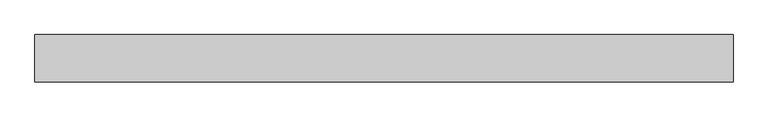
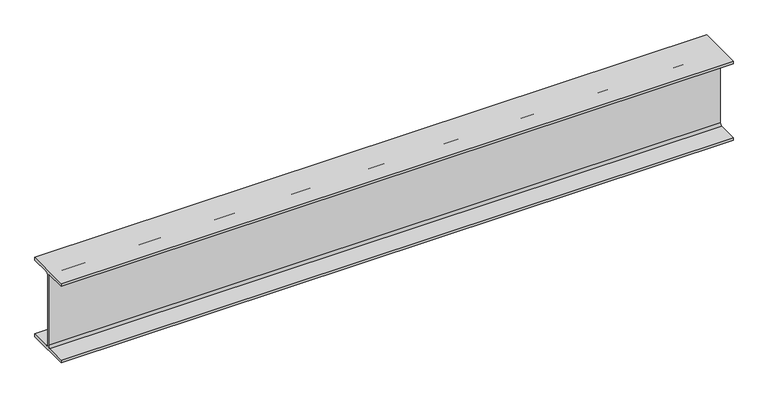
"""IFC4 building model written with IfcOpenShell, lengths in millimetres: beam geometry, Steel Beam_H-KSD3502 : H_SB_ASB_H-194x150x6x9."""

import ifcopenshell
import ifcopenshell.guid

model = None  # the IFC model being written
_history = None  # IfcOwnerHistory: only IFC2X3 demands one
_inside = {}  # id of a spatial element -> (the spatial element, [elements in it])
_under = {}  # id of a project, library or spatial element -> (it, [spatial elements below it])
_declared = {}  # id of a project -> (the project, [libraries it declares])
_typed = {}  # id of a type object -> (the type object, [elements of that type])
_made_of = {}  # id of a material, layer set ... -> (it, [elements and type objects made of it])


def new_model(schema):
    """Start an empty IFC model of exactly this schema.

    Asked for "IFC4X3", IfcOpenShell would pick the latest addendum, in which some entities
    have other attributes; the version numbers below select the first issue.
    IFC2X3 requires an IfcOwnerHistory on every rooted entity: one is made here for all.
    """
    global model, _history
    if schema == "IFC4X3":
        model = ifcopenshell.file(schema_version=(4, 3, 0, 0))
    else:
        model = ifcopenshell.file(schema=schema)
    _inside.clear()
    _under.clear()
    _declared.clear()
    _typed.clear()
    _made_of.clear()
    _history = None
    if model.schema == "IFC2X3":
        org = make("IfcOrganization", Name="unknown")
        user = make(
            "IfcPersonAndOrganization",
            ThePerson=make("IfcPerson", FamilyName="unknown"),
            TheOrganization=org,
        )
        app = make(
            "IfcApplication",
            ApplicationDeveloper=org,
            Version="unknown",
            ApplicationFullName="unknown",
            ApplicationIdentifier="unknown",
        )
        _history = make(
            "IfcOwnerHistory",
            OwningUser=user,
            OwningApplication=app,
            ChangeAction="ADDED",
            CreationDate=0,
        )
    return model


def make(cls, **values):
    """One entity of the class cls with the attributes given. An attribute that is None is left unset."""
    return model.create_entity(
        cls, **{name: value for name, value in values.items() if value is not None}
    )


def rooted(cls, **values):
    """An entity with a GlobalId (a new one), such as an element, a storey or a relation."""
    return make(cls, GlobalId=ifcopenshell.guid.new(), OwnerHistory=_history, **values)


def si_unit(unit_type, name, prefix=None):
    """IfcSIUnit, for example si_unit("LENGTHUNIT", "METRE", prefix="MILLI")."""
    return make("IfcSIUnit", UnitType=unit_type, Prefix=prefix, Name=name)


def assignment(units):
    """IfcUnitAssignment: the units of a project."""
    return None if units is None else make("IfcUnitAssignment", Units=units)


def point(xyz):
    """IfcCartesianPoint."""
    return None if xyz is None else make("IfcCartesianPoint", Coordinates=xyz)


def direction(xyz):
    """IfcDirection."""
    return None if xyz is None else make("IfcDirection", DirectionRatios=xyz)


def frame(location, z_axis=None, x_axis=None):
    """IfcAxis2Placement3D, a coordinate frame: its origin and axes. An axis left out is left unset."""
    return make(
        "IfcAxis2Placement3D",
        Location=point(location),
        Axis=direction(z_axis),
        RefDirection=direction(x_axis),
    )


def frame_2d(location, x_axis=None):
    """IfcAxis2Placement2D, a coordinate frame in the plane: its origin and x axis."""
    return make(
        "IfcAxis2Placement2D", Location=point(location), RefDirection=direction(x_axis)
    )


def origin():
    """The frame at (0, 0, 0) with its axes left unset."""
    return frame((0.0, 0.0, 0.0))


def place(relative_to, where):
    """IfcLocalPlacement: puts the frame where relative to a parent placement (None: the world)."""
    return make(
        "IfcLocalPlacement", PlacementRelTo=relative_to, RelativePlacement=where
    )


def context(
    kind, dimensions, precision=None, world=None, true_north=None, identifier=None
):
    """IfcGeometricRepresentationContext, for example the 3D "Model" context."""
    return make(
        "IfcGeometricRepresentationContext",
        ContextIdentifier=identifier,
        ContextType=kind,
        CoordinateSpaceDimension=dimensions,
        Precision=precision,
        WorldCoordinateSystem=world,
        TrueNorth=true_north,
    )


def project(units=None, contexts=None):
    """IfcProject with its units and contexts."""
    return rooted(
        "IfcProject",
        Name="project",
        RepresentationContexts=contexts,
        UnitsInContext=assignment(units),
    )


def spatial(cls, under=None, at=None, **own):
    """A site, building, storey or space (cls), placed at a placement, below another one or the project."""
    s = rooted(cls, ObjectPlacement=at, **own)
    if under is not None:
        _under.setdefault(under.id(), (under, []))[1].append(s)
    return s


def polyline(points):
    """IfcPolyline through the points."""
    return make("IfcPolyline", Points=[point(p) for p in points])


def circle_curve(where, radius):
    """IfcCircle in the frame where."""
    return make("IfcCircle", Position=where, Radius=radius)


def trimmed(basis, trim1, trim2, sense, master):
    """IfcTrimmedCurve: the piece of a basis curve between two trims."""
    return make(
        "IfcTrimmedCurve",
        BasisCurve=basis,
        Trim1=trim1,
        Trim2=trim2,
        SenseAgreement=sense,
        MasterRepresentation=master,
    )


def segment(curve, same_sense, transition):
    """IfcCompositeCurveSegment."""
    return make(
        "IfcCompositeCurveSegment",
        Transition=transition,
        SameSense=same_sense,
        ParentCurve=curve,
    )


def composite_curve(segments, self_intersect=None):
    """IfcCompositeCurve: segments joined end to end."""
    return make("IfcCompositeCurve", Segments=segments, SelfIntersect=self_intersect)


def outline(outer, holes=None, kind="AREA"):
    """IfcArbitraryClosedProfileDef: a profile drawn as a closed curve; with holes, ...WithVoids."""
    if holes is None:
        return make("IfcArbitraryClosedProfileDef", ProfileType=kind, OuterCurve=outer)
    return make(
        "IfcArbitraryProfileDefWithVoids",
        ProfileType=kind,
        OuterCurve=outer,
        InnerCurves=holes,
    )


def extrude(swept, where, along, depth):
    """IfcExtrudedAreaSolid: the profile swept, set in the frame where, extruded along a direction by depth."""
    return make(
        "IfcExtrudedAreaSolid",
        SweptArea=swept,
        Position=where,
        ExtrudedDirection=direction(along),
        Depth=depth,
    )


def shape(context_of_items, identifier, shape_type, items):
    """IfcShapeRepresentation: the items that make up one representation, for example the "Body"."""
    return make(
        "IfcShapeRepresentation",
        ContextOfItems=context_of_items,
        RepresentationIdentifier=identifier,
        RepresentationType=shape_type,
        Items=items,
    )


def source(mapping_origin, context_of_items, identifier, shape_type, items):
    """IfcRepresentationMap: a shape defined once, which mapped items show again and again."""
    return make(
        "IfcRepresentationMap",
        MappingOrigin=mapping_origin,
        MappedRepresentation=shape(context_of_items, identifier, shape_type, items),
    )


def transform(
    local_origin,
    x_axis=None,
    y_axis=None,
    z_axis=None,
    scale=None,
    scale2=None,
    scale3=None,
    uniform=True,
):
    """IfcCartesianTransformationOperator3D, or its non-uniform kind. x_axis, y_axis, z_axis: its Axis1, 2, 3."""
    if uniform:
        return make(
            "IfcCartesianTransformationOperator3D",
            Axis1=direction(x_axis),
            Axis2=direction(y_axis),
            LocalOrigin=point(local_origin),
            Scale=scale,
            Axis3=direction(z_axis),
        )
    return make(
        "IfcCartesianTransformationOperator3DnonUniform",
        Axis1=direction(x_axis),
        Axis2=direction(y_axis),
        LocalOrigin=point(local_origin),
        Scale=scale,
        Axis3=direction(z_axis),
        Scale2=scale2,
        Scale3=scale3,
    )


def mapped(mapping_source, mapping_target):
    """IfcMappedItem: shows the shape of a source again, moved by a transform."""
    return make(
        "IfcMappedItem", MappingSource=mapping_source, MappingTarget=mapping_target
    )


def made_of(thing, what):
    """Note that an element or type object is made of a material, layer set ...; save() writes the relation."""
    if what is not None:
        _made_of.setdefault(what.id(), (what, []))[1].append(thing)
    return thing


def element(
    cls,
    number,
    at=None,
    inside=None,
    cuts=None,
    type_object=None,
    material=None,
    context=None,
    identifier="Body",
    shape_type=None,
    held_by="IfcProductDefinitionShape",
    body=None,
    shapes=None,
    **own,
):
    """One element of the class cls, such as IfcWall. Its Tag is "e" and its number.

    at: its placement. inside: the storey or other place that contains it. cuts: it is an
    opening in that element (IfcRelVoidsElement). A single representation is given by context,
    identifier, shape_type and body (its items); several are given by shapes. held_by: the class
    of the entity that holds the representations. save() writes the other relations.
    """
    e = rooted(cls, Tag="e%d" % number, ObjectPlacement=at, **own)
    if body is not None:
        shapes = [shape(context, identifier, shape_type, body)]
    if shapes is not None:
        e.Representation = make(held_by, Representations=shapes)
    if inside is not None:
        _inside.setdefault(inside.id(), (inside, []))[1].append(e)
    if cuts is not None:
        rooted(
            "IfcRelVoidsElement", RelatingBuildingElement=cuts, RelatedOpeningElement=e
        )
    if type_object is not None:
        _typed.setdefault(type_object.id(), (type_object, []))[1].append(e)
    return made_of(e, material)


def aggregate(whole, parts):
    """IfcRelAggregates: a whole, such as a stair, and the parts it consists of."""
    return rooted("IfcRelAggregates", RelatingObject=whole, RelatedObjects=parts)


def save(model, path):
    """Write the relations noted so far, then the file.

    IfcRelAggregates (storeys below a building ...), IfcRelContainedInSpatialStructure (elements
    in a storey), IfcRelDefinesByType, IfcRelAssociatesMaterial and IfcRelDeclares: one each for
    every whole, place, type object, material and project.
    """
    for whole, parts in _under.values():
        aggregate(whole, parts)
    for where, things in _inside.values():
        rooted(
            "IfcRelContainedInSpatialStructure",
            RelatedElements=things,
            RelatingStructure=where,
        )
    for kind, things in _typed.values():
        rooted("IfcRelDefinesByType", RelatedObjects=things, RelatingType=kind)
    for what, things in _made_of.values():
        rooted("IfcRelAssociatesMaterial", RelatedObjects=things, RelatingMaterial=what)
    for by, libraries in _declared.values():
        rooted("IfcRelDeclares", RelatingContext=by, RelatedDefinitions=libraries)
    model.write(path)


def beam_16990a11(model_context):
    return source(origin(), model_context, "Body", "SweptSolid", [
        extrude(outline(composite_curve([segment(polyline([(-82.5, -141.5), (-11.9, -141.5)]), True, "CONTINUOUS"), segment(trimmed(circle_curve(frame_2d((-11.9, -132.6)), 8.9), [point((-11.9, -141.5))], [point((-3.0, -132.6))], True, "CARTESIAN"), True, "CONTINUOUS"), segment(polyline([(-3.0, -132.6), (-3.0, 132.6)]), True, "CONTINUOUS"), segment(trimmed(circle_curve(frame_2d((-11.9, 132.6)), 8.9), [point((-3.0, 132.6))], [point((-11.9, 141.5))], True, "CARTESIAN"), True, "CONTINUOUS"), segment(polyline([(-11.9, 141.5), (-82.5, 141.5), (-82.5, 151.7), (82.5, 151.7), (82.5, 141.5), (11.9, 141.5)]), True, "CONTINUOUS"), segment(trimmed(circle_curve(frame_2d((11.9, 132.6)), 8.9), [point((11.9, 141.5))], [point((3.0, 132.6))], True, "CARTESIAN"), True, "CONTINUOUS"), segment(polyline([(3.0, 132.6), (3.0, -132.6)]), True, "CONTINUOUS"), segment(trimmed(circle_curve(frame_2d((11.9, -132.6)), 8.9), [point((3.0, -132.6))], [point((11.9, -141.5))], True, "CARTESIAN"), True, "CONTINUOUS"), segment(polyline([(11.9, -141.5), (82.5, -141.5), (82.5, -151.7), (-82.5, -151.7), (-82.5, -141.5)]), True, "CONTINUOUS")], self_intersect=False)), frame((-1200.0, 0.0, 0.0), z_axis=(1.0, 0.0, 0.0), x_axis=(0.0, 1.0, 0.0)), (0.0, 0.0, 1.0), 2433.3704936),
    ])


if __name__ == "__main__":
    model = new_model("IFC4")
    model_context = context("Model", 3, world=origin())
    ifc_project = project(units=[si_unit("LENGTHUNIT", "METRE", prefix="MILLI")], contexts=[model_context])
    site = spatial("IfcSite", under=ifc_project)
    building = spatial("IfcBuilding", under=site)
    placement = place(None, origin())
    beam_shape = beam_16990a11(model_context)
    element("IfcBeam", 1, ObjectType="Steel Beam_H-KSD3502 : H_SB_ASB_H-194x150x6x9", at=placement, inside=building, context=model_context, shape_type="MappedRepresentation", body=[
        mapped(beam_shape, transform((0.0, 0.0, 0.0), x_axis=(1.0, 0.0, 0.0), y_axis=(0.0, 1.0, 0.0), z_axis=(0.0, 0.0, 1.0))),
    ])
    save(model, "model.ifc")

# Revit data of these elements
# Type "Steel Beam_H-KSD3502 : H_SB_ASB_H-194x150x6x9"
#   Width = 15.0 cm
#   Web Thickness = 0.6 cm
#   Web Fillet = 1.3 cm
#   Warping Constant = 43316.0 cm⁶
#   Torsional Moment of Inertia = 8.622 cm⁴
#   Torsional Modulus = 1.0 cm³
#   Section Area = 39.01 cm²
#   Plastic Modulus weak axis = 104.0 cm³
#   Plastic Modulus strong axis = 309.0 cm³
#   Perimeter = 0.95 m²/m
#   Nominal Weight = 30.60 kgf/m
#   Moment of Inertia weak axis = 507.00 cm⁴
#   Moment of Inertia strong axis = 2690.00 cm⁴
#   Height = 19.4 cm
#   Flange Thickness = 0.9 cm
#   Elastic Modulus weak axis = 67.6 cm³
#   Elastic Modulus strong axis = 277.0 cm³
#   Centroid Vertical = 9.7 cm
#   Centroid Horizontal = 7.5 cm
#   Length [instance default] = 1.5240 m
#   Structural Material [instance default] = Steel, 45-345
#   Assembly Code = ""
# Element 1 (IfcBeam, "Steel Beam_H-KSD3502 : H_SB_ASB_H-194x150x6x9")
#   Structural Material = none
# Materials
#   "Steel, 45-345": class "Metal", colour RGB 189 187 185, transparency 0, Description = "Steel 345 MPa", Cost = 0
